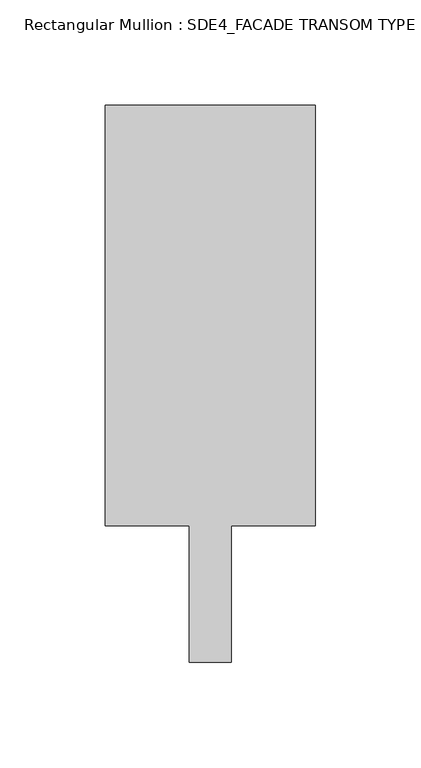
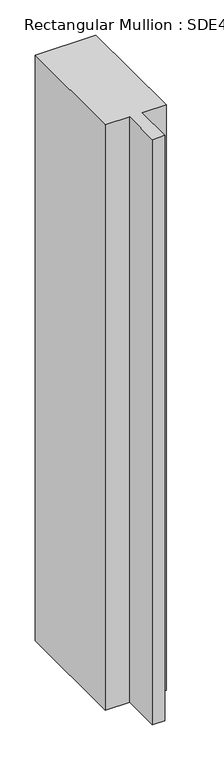
"""IFC4 building model written with IfcOpenShell, lengths in millimetres: member geometry, Rectangular Mullion : SDE4_FACADE TRANSOM TYPE 2."""

from ifc_helpers import new_model, si_unit, frame, origin, place, context, project, spatial, polyline, outline, extrude, source, transform, mapped, element, save


def rectangular_mullion_sde4_facade_transom_type_2_47438292(model_context):
    return source(origin(), model_context, "Body", "SweptSolid", [
        extrude(outline(polyline([(50.0, 132.5), (50.0, -67.5), (10.0, -67.5), (10.0, -132.5), (-10.0, -132.5), (-10.0, -67.5), (-50.0, -67.5), (-50.0, 132.5), (50.0, 132.5)])), frame((0.0, 0.0, -1018.375), z_axis=(0.0, 0.0, 1.0), x_axis=(1.0, 0.0, 0.0)), (0.0, 0.0, 1.0), 1018.375),
    ])


if __name__ == "__main__":
    model = new_model("IFC4")
    model_context = context("Model", 3, world=origin())
    ifc_project = project(units=[si_unit("LENGTHUNIT", "METRE", prefix="MILLI")], contexts=[model_context])
    site = spatial("IfcSite", under=ifc_project)
    building = spatial("IfcBuilding", under=site)
    placement = place(None, origin())
    rectangular_mullion_sde4_facade_transom_type_2_shape = rectangular_mullion_sde4_facade_transom_type_2_47438292(model_context)
    element("IfcMember", 1, ObjectType="Rectangular Mullion : SDE4_FACADE TRANSOM TYPE 2", at=placement, inside=building, context=model_context, shape_type="MappedRepresentation", body=[
        mapped(rectangular_mullion_sde4_facade_transom_type_2_shape, transform((0.0, 0.0, 0.0), x_axis=(1.0, 0.0, 0.0), y_axis=(0.0, 1.0, 0.0), z_axis=(0.0, 0.0, 1.0))),
    ])
    save(model, "model.ifc")

# Revit data of these elements
# Type "Rectangular Mullion : SDE4_FACADE TRANSOM TYPE 2"
#   built-in parameter 1007322 = 0.869423 (stored number, unit not read)
#   built-in parameter 1007321 = 0.164042 (stored number, unit not read)
#   built-in parameter 1007320 = 0.164042 (stored number, unit not read)
